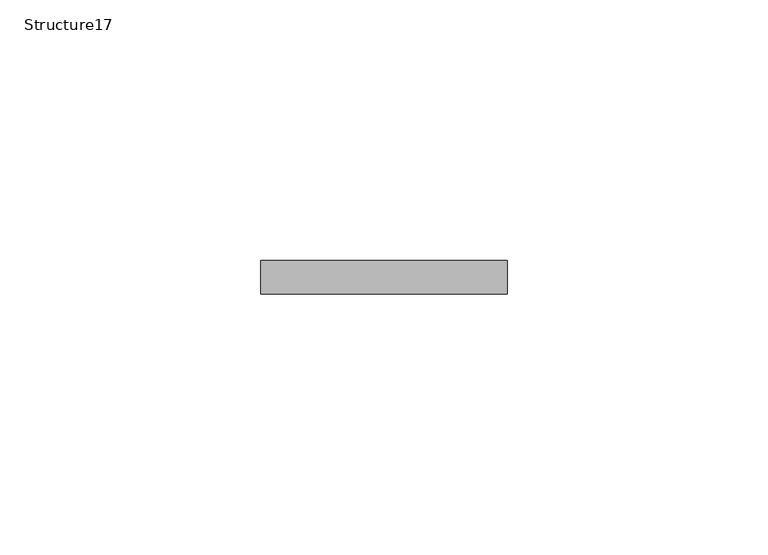
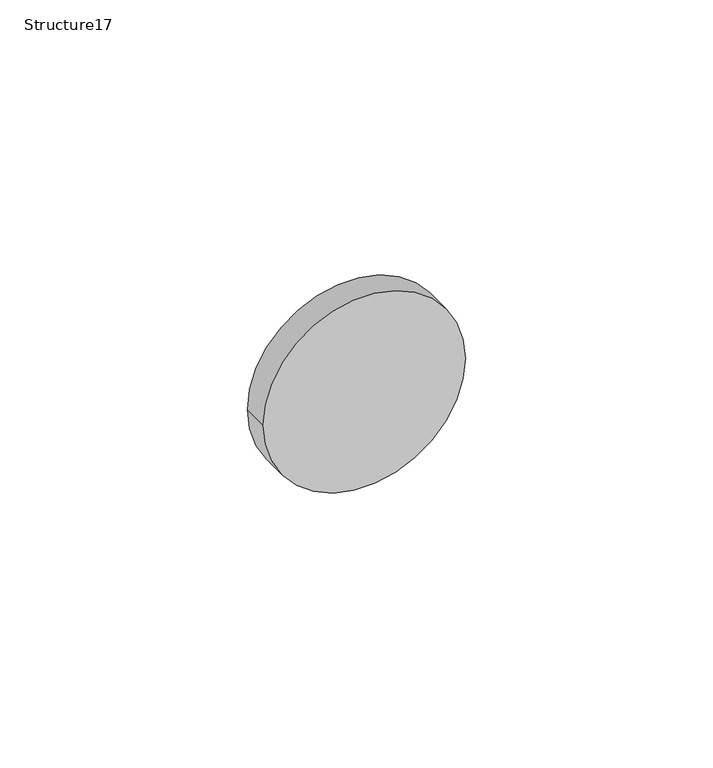
"""IFC4 building model written with IfcOpenShell, lengths in millimetres: proxy geometry, Structure17 : Structure668217138."""

from ifc_helpers import new_model, si_unit, point, frame, frame_2d, origin, place, context, project, spatial, circle_curve, trimmed, segment, composite_curve, outline, extrude, source, transform, mapped, element, save


def structure17_c8fa977f(model_context):
    return source(origin(), model_context, "Body", "SweptSolid", [
        extrude(outline(composite_curve([segment(trimmed(circle_curve(frame_2d((39371.6422813, 7343.0332877)), 23.5716554), [point((39371.6422813, 7319.4616323))], [point((39371.6422813, 7366.6049431))], False, "CARTESIAN"), True, "CONTINUOUS"), segment(trimmed(circle_curve(frame_2d((39371.6422813, 7343.0332877)), 23.5716554), [point((39371.6422813, 7366.6049431))], [point((39371.6422813, 7319.4616323))], False, "CARTESIAN"), True, "CONTINUOUS")], self_intersect=False)), frame((0.0, 1959.9461961, 0.0), z_axis=(0.0, 1.0, 0.0), x_axis=(0.0, 0.0, 1.0)), (0.0, 0.0, 1.0), 6.35),
    ])


if __name__ == "__main__":
    model = new_model("IFC4")
    model_context = context("Model", 3, world=origin())
    ifc_project = project(units=[si_unit("LENGTHUNIT", "METRE", prefix="MILLI")], contexts=[model_context])
    site = spatial("IfcSite", under=ifc_project)
    building = spatial("IfcBuilding", under=site)
    placement = place(None, origin())
    structure17_shape = structure17_c8fa977f(model_context)
    element("IfcBuildingElementProxy", 1, Name="Structure17 : Structure668217138", ObjectType="Structure17 : Structure668217138", at=placement, inside=building, context=model_context, shape_type="MappedRepresentation", body=[
        mapped(structure17_shape, transform((0.0, 0.0, 0.0), x_axis=(1.0, 0.0, 0.0), y_axis=(0.0, 1.0, 0.0), z_axis=(0.0, 0.0, 1.0))),
    ])
    save(model, "model.ifc")

# Revit data of these elements
# Type "Structure17 : Structure668217138"
#   NameOverride = "Structure668217138"
# Element 1 (IfcBuildingElementProxy, "Structure17 : Structure668217138")
#   Materials on its faces: "RUBBER GASKET"
# Materials
#   "RUBBER GASKET": class "Unassigned", colour RGB 70 70 70, transparency 0
